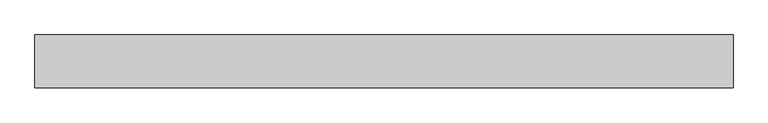
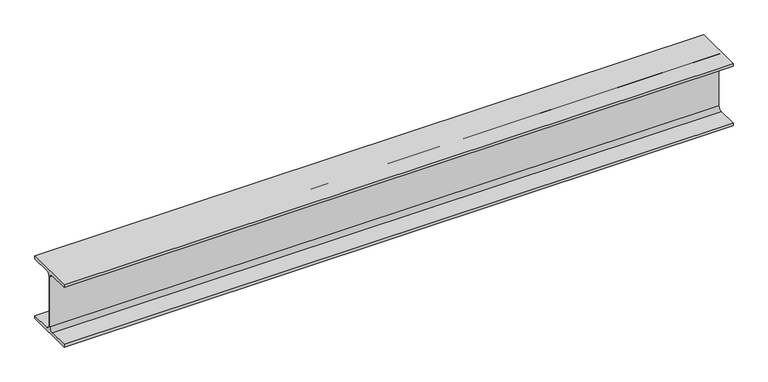
"""IFC4 building model written with IfcOpenShell, lengths in millimetres: beam geometry, 0912_Steel Framing_H-KSD3502 : H_SB_ASB_H-390x300x10x16."""

from ifc_helpers import new_model, si_unit, point, frame, frame_2d, origin, place, context, project, spatial, polyline, circle_curve, trimmed, segment, composite_curve, outline, extrude, source, transform, mapped, element, save


def beam_ba909a4e(model_context):
    return source(origin(), model_context, "Body", "SweptSolid", [
        extrude(outline(composite_curve([segment(polyline([(150.0, -179.0), (150.0, -195.0), (-150.0, -195.0), (-150.0, -179.0), (-27.0, -179.0)]), True, "CONTINUOUS"), segment(trimmed(circle_curve(frame_2d((-27.0, -157.0)), 22.0), [point((-27.0, -179.0))], [point((-5.0, -157.0))], True, "CARTESIAN"), True, "CONTINUOUS"), segment(polyline([(-5.0, -157.0), (-5.0, 157.0)]), True, "CONTINUOUS"), segment(trimmed(circle_curve(frame_2d((-27.0, 157.0)), 22.0), [point((-5.0, 157.0))], [point((-27.0, 179.0))], True, "CARTESIAN"), True, "CONTINUOUS"), segment(polyline([(-27.0, 179.0), (-150.0, 179.0), (-150.0, 195.0), (150.0, 195.0), (150.0, 179.0), (27.0, 179.0)]), True, "CONTINUOUS"), segment(trimmed(circle_curve(frame_2d((27.0, 157.0)), 22.0), [point((27.0, 179.0))], [point((5.0, 157.0))], True, "CARTESIAN"), True, "CONTINUOUS"), segment(polyline([(5.0, 157.0), (5.0, -157.0)]), True, "CONTINUOUS"), segment(trimmed(circle_curve(frame_2d((27.0, -157.0)), 22.0), [point((5.0, -157.0))], [point((27.0, -179.0))], True, "CARTESIAN"), True, "CONTINUOUS"), segment(polyline([(27.0, -179.0), (150.0, -179.0)]), True, "CONTINUOUS")], self_intersect=False)), frame((-1987.2999994, 0.0, 0.0), z_axis=(1.0, 0.0, 0.0), x_axis=(0.0, 1.0, 0.0)), (0.0, 0.0, 1.0), 3974.5999988),
    ])


if __name__ == "__main__":
    model = new_model("IFC4")
    model_context = context("Model", 3, world=origin())
    ifc_project = project(units=[si_unit("LENGTHUNIT", "METRE", prefix="MILLI")], contexts=[model_context])
    site = spatial("IfcSite", under=ifc_project)
    building = spatial("IfcBuilding", under=site)
    placement = place(None, origin())
    beam_shape = beam_ba909a4e(model_context)
    element("IfcBeam", 1, ObjectType="0912_Steel Framing_H-KSD3502 : H_SB_ASB_H-390x300x10x16", at=placement, inside=building, context=model_context, shape_type="MappedRepresentation", body=[
        mapped(beam_shape, transform((0.0, 0.0, 0.0), x_axis=(1.0, 0.0, 0.0), y_axis=(0.0, 1.0, 0.0), z_axis=(0.0, 0.0, 1.0))),
    ])
    save(model, "model.ifc")

# Revit data of these elements
# Type "0912_Steel Framing_H-KSD3502 : H_SB_ASB_H-390x300x10x16"
#   H_WM Code_1 = "S01AA001-00001 | Main Steel Structure Fabrication Work | Shelter/Building | Heavy Steel - Standard (Weight≥90KG/M) | Material: (   )"
#   H_WM Code_2 = "S03AA027-00001 | Main Steel Structure Erection Work | Shelter/Building | Heavy Steel (Weight≥90KG/M) | Material: (   )"
#   H_WM Code_3 = "S01AA010-00001 | Main Steel Structure Fabrication Work | Shelter/Building | Steel Painting/Coating | for Non-Fireproofed Steel Surface, Surface Preparation, Primer, Second & Final Coat | Material: (   )"
#   H_Q'ty Cal Type Tag = "SB-Q2"
#   Width = 30.0 cm
#   Web Thickness = 1.0 cm
#   Web Fillet = 2.2 cm
#   Warping Constant = 2520000.0 cm⁶
#   W = 0
#   Torsional Moment of Inertia = 94.3867 cm⁴
#   Section Area = 136.0 cm²
#   Plastic Modulus weak axis = 733.0 cm³
#   Plastic Modulus strong axis = 2190.0 cm³
#   Perimeter = 1.92 m²/m
#   Nominal Weight = 107.00 kgf/m
#   Moment of Inertia weak axis = 7210.00 cm⁴
#   Moment of Inertia strong axis = 38700.00 cm⁴
#   Height = 39.0 cm
#   Flange Thickness = 1.6 cm
#   Elastic Modulus weak axis = 481.0 cm³
#   Elastic Modulus strong axis = 1980.0 cm³
#   Centroid Vertical = 19.5 cm
#   Centroid Horizontal = 15.0 cm
#   Ix = 387000000
#   Length [instance default] = 1.5240 m
#   Zx = 2190000
#   b = 0.3000 m
#   h = 0.3900 m
#   r = 0.0220 m
#   s = 0.0100 m
#   t = 0.0160 m
#   A = 0.0136 m²
#   Structural Material [instance default] = Steel, 45-345
#   Assembly Code = ""
# Element 1 (IfcBeam, "0912_Steel Framing_H-KSD3502 : H_SB_ASB_H-390x300x10x16")
#   Structural Material = none
# Materials
#   "Steel, 45-345": class "Metal", colour RGB 189 187 185, transparency 0, Description = "Steel 345 MPa", Cost = 0
